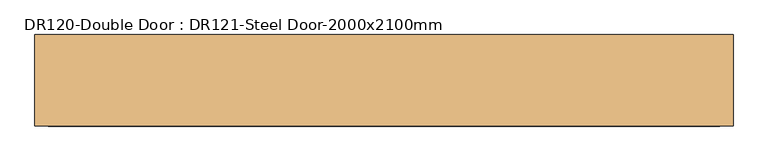
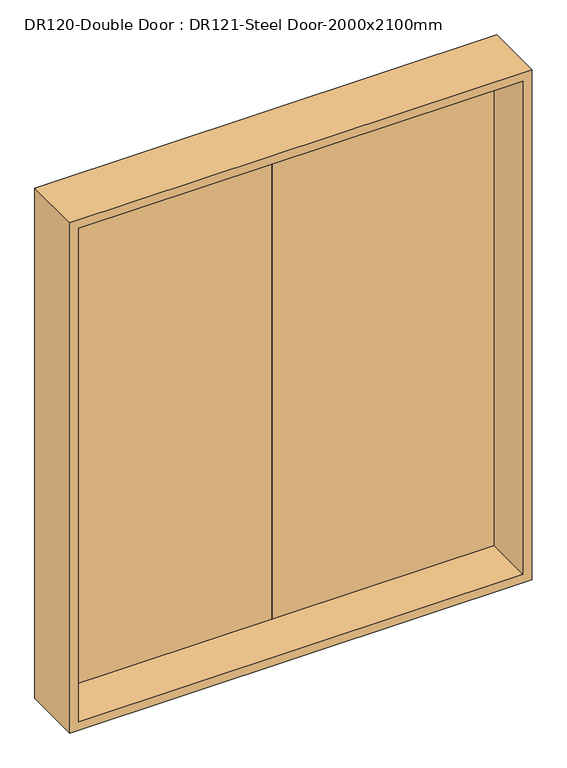
"""IFC4 building model written with IfcOpenShell, lengths in millimetres: door geometry, DR120-Double Door : DR121-Steel Door-2000x2100mm."""

from ifc_helpers import new_model, si_unit, frame, origin, place, context, project, spatial, polyline, outline, extrude, faceted_brep, source, transform, mapped, element, save


def dr120_double_door_dr121_steel_door_2000x2100mm_b13dcabf(model_context):
    return source(origin(), model_context, "Body", "SolidModel", [
        extrude(outline(polyline([(880.0, 78.0), (0.0, 78.0), (0.0, 118.0), (880.0, 118.0), (880.0, 78.0)])), frame((0.0, 0.0, 20.0), z_axis=(0.0, 0.0, 1.0), x_axis=(1.0, 0.0, 0.0)), (0.0, 0.0, 1.0), 2060.0),
        extrude(outline(polyline([(0.0, 78.0), (-880.0, 78.0), (-880.0, 118.0), (0.0, 118.0), (0.0, 78.0)])), frame((0.0, 0.0, 20.0), z_axis=(0.0, 0.0, 1.0), x_axis=(1.0, 0.0, 0.0)), (0.0, 0.0, 1.0), 2060.0),
        faceted_brep([(900.0, -118.0, 2100.0), (900.0, 118.0, 2100.0), (-900.0, 118.0, 2100.0), (-900.0, -118.0, 2100.0), (865.0, 78.0, 2065.0), (865.0, -118.0, 2065.0), (-865.0, -118.0, 2065.0), (-865.0, 78.0, 2065.0), (880.0, 118.0, 2080.0), (880.0, 78.0, 2080.0), (-880.0, 78.0, 2080.0), (-880.0, 118.0, 2080.0), (-900.0, 118.0, 0.0), (-900.0, -118.0, 0.0), (-865.0, -118.0, 35.0), (-865.0, 78.0, 35.0), (-880.0, 78.0, 20.0), (-880.0, 118.0, 20.0), (900.0, 118.0, 0.0), (880.0, 118.0, 20.0), (900.0, -118.0, 0.0), (865.0, -118.0, 35.0), (865.0, 78.0, 35.0), (880.0, 78.0, 20.0)], [[[0, 1, 2, 3]], [[4, 5, 6, 7]], [[8, 9, 10, 11]], [[3, 2, 12, 13]], [[7, 6, 14, 15]], [[11, 10, 16, 17]], [[18, 12, 2, 1], [8, 11, 17, 19]], [[13, 12, 18, 20]], [[0, 3, 13, 20], [21, 14, 6, 5]], [[15, 14, 21, 22]], [[23, 16, 10, 9], [4, 7, 15, 22]], [[17, 16, 23, 19]], [[20, 18, 1, 0]], [[22, 21, 5, 4]], [[19, 23, 9, 8]]]),
    ])


if __name__ == "__main__":
    model = new_model("IFC4")
    model_context = context("Model", 3, world=origin())
    ifc_project = project(units=[si_unit("LENGTHUNIT", "METRE", prefix="MILLI")], contexts=[model_context])
    site = spatial("IfcSite", under=ifc_project)
    building = spatial("IfcBuilding", under=site)
    placement = place(None, origin())
    dr120_double_door_dr121_steel_door_2000x2100mm_shape = dr120_double_door_dr121_steel_door_2000x2100mm_b13dcabf(model_context)
    element("IfcDoor", 1, ObjectType="DR120-Double Door : DR121-Steel Door-2000x2100mm", at=placement, inside=building, context=model_context, shape_type="MappedRepresentation", body=[
        mapped(dr120_double_door_dr121_steel_door_2000x2100mm_shape, transform((0.0, 0.0, 0.0), x_axis=(1.0, 0.0, 0.0), y_axis=(0.0, 1.0, 0.0), z_axis=(0.0, 0.0, 1.0))),
    ])
    save(model, "model.ifc")

# Revit data of these elements
# Type "DR120-Double Door : DR121-Steel Door-2000x2100mm"
#   Type Mark = "SD"
#   프레임 = ""
#   철물 = ""
#   유리/마감 = ""
#   위치/개소 = ""
#   부호 = "1/SD"
#   문번호 = ""
#   문기호 = "SD"
#   Analytic Construction = "<None>"
#   Height = 2100 mm
#   Width = 1800 mm
#   Define Thermal Properties by = 1
#   문 틀 = A04AQ098-00003_Steel Door_non FP_double
#   문 = 문
#   Function = (empty or 0)
#   Assembly Code = ""
#   Wall Closure = (empty or 0)
# Element 1 (IfcDoor, "DR120-Double Door : DR121-Steel Door-2000x2100mm")
#   Materials on its faces: "A04AQ098-00003_Steel Door_non FP_double", "문"
# Materials
#   "A04AQ098-00003_Steel Door_non FP_double": class "금속", colour RGB 247 247 247, transparency 0, Description = "Steel Door", W00) Work Master Code = "A04AQ098-00003", W01) Work Master_Lv1 = "Finishing Work", W02) Work Master_Lv2 = "Door & Window Work", W03) Work Master_Spec.1 = "Steel Door w/ Steel Frame", W04) Work Master_Spec.2 = "Fire Protective Rating: N/A, Double Door", W05) Work Master_Spec.3 = "w/ Hardware & Accessories", Cost = 0
#   "문": class "다양한", colour RGB 247 247 247, transparency 0
